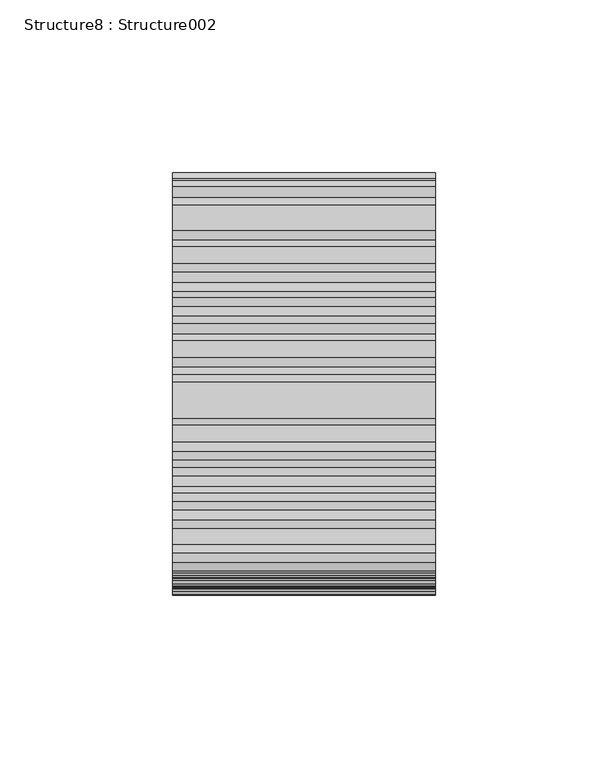
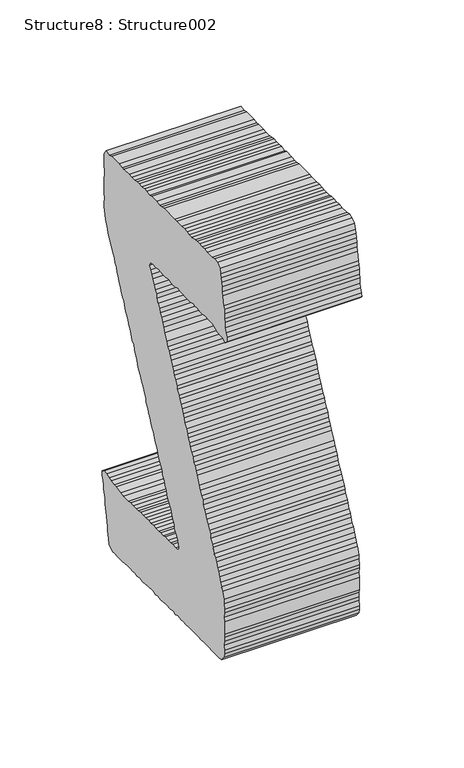
"""IFC4 building model written with IfcOpenShell, lengths in millimetres: proxy geometry, Structure8 : Structure002."""

from ifc_helpers import new_model, si_unit, frame, origin, place, context, project, spatial, polyline, outline, extrude, source, transform, mapped, element, save


def structure8_structure002_856189c6(model_context):
    return source(origin(), model_context, "Body", "SweptSolid", [
        extrude(outline(polyline([(2.492598, 0.0), (3.6086259, -2.5762556), (4.2959642, -5.0304922), (4.9764723, -7.4847267), (6.2027504, -9.6321841), (6.7842527, -12.5126982), (7.5898251, -14.5452844), (8.7003896, -17.1188063), (9.3874124, -19.5741986), (10.0456375, -21.3367914), (10.7326603, -23.7921837), (11.6960865, -26.0994951), (12.9542114, -28.9331331), (14.0275724, -30.8128021), (14.7236303, -33.2737663), (15.5292027, -35.3063524), (16.5191192, -38.292172), (14.6444913, -41.866959), (12.6028699, -42.6669596), (10.8807391, -44.0162015), (6.0473046, -46.7762723), (1.4407763, -48.6916737), (-0.4433067, -49.7675552), (-2.7074205, -51.4097046), (-5.0096886, -52.375129), (-6.3099559, -53.8327276), (-8.7690266, -54.5218508), (-11.1433905, -56.5927984), (-16.0213856, -58.6632174), (-20.0485121, -60.9628564), (-21.8924489, -62.7309104), (-24.0800527, -63.265016), (-26.1866282, -65.1830464), (-28.6055525, -66.5643422), (-30.9149624, -67.5172599), (-34.9457673, -69.8189993), (-37.510674, -70.9344002), (-39.0824083, -72.5470164), (-41.2744262, -73.0836426), (-43.6487901, -75.1545902), (-45.9574643, -76.1070878), (-48.219586, -77.7646846), (-50.5238461, -78.7146616), (-58.5869273, -83.3189807), (-61.110952, -85.1261339), (-62.8811066, -85.7711168), (-67.4519025, -88.3812112), (-69.4366719, -89.8804296), (-75.6193484, -93.4109677), (-78.4635995, -94.6692996), (-81.7199432, -93.3318287), (-83.4889419, -91.4845292), (-84.5581018, -89.6122169), (-85.4008779, -86.8857779), (-86.8984097, -84.8834606), (-88.1246878, -82.7360031), (-89.3170185, -81.2784046), (-93.0000537, -74.8286753), (-93.6857117, -72.3773815), (-95.753403, -70.0070116), (-96.6809884, -68.3826244), (-97.6720606, -65.3964894), (-98.9025397, -63.2416751), (-99.9709638, -58.8763448), (-100.0929769, -56.7919458), (-100.0855196, -54.3106986), (-100.5064322, -51.6926162), (-101.0804771, -48.823453), (-100.7731694, -46.8587615), (-101.3546716, -43.9782474), (-101.8848918, -41.7991562), (-101.3113735, -39.6873265), (-102.0372804, -36.5351385), (-102.2773205, -34.883003), (-101.8888818, -31.8183601), (-102.8432728, -29.5166206), (-102.8007104, -27.7187177), (-103.1167317, -24.670995), (-102.8433774, -22.0369352), (-103.1067517, -19.6947337), (-103.1096945, -17.2038161), (-103.1016019, -14.706597), (-104.2213082, -12.1324419), (-103.9075945, -10.1806771), (-104.0688112, -7.4142986), (-104.2129002, -4.648871), (-104.6411697, 0.4576085), (-104.9043371, 2.7891968), (-105.1715969, 5.1399108), (-104.8677605, 7.0918886), (-105.7105366, 9.8183277), (-105.2863656, 12.1882775), (-105.4431682, 14.9571766), (-105.9772738, 17.1447805), (-105.9730728, 19.6300217), (-106.087944, 21.701914), (-106.507914, 24.3098034), (-106.3936699, 27.2344558), (-106.8132196, 29.8416095), (-106.934497, 31.9264286), (-107.624569, 34.3752018), (-107.6189991, 36.8700049), (-107.7719163, 39.6303914), (-108.0012408, 41.2740122), (-107.6219398, 44.3529487), (-108.2634594, 46.1084961), (-108.3049706, 49.2973651), (-108.1557299, 51.5269043), (-108.6898354, 53.7145081), (-108.9617224, 56.0528242), (-108.9931492, 59.230867), (-109.2673436, 61.5834745), (-109.6852131, 64.1876855), (-109.1029752, 66.2927875), (-109.9522658, 69.0203844), (-109.9070742, 73.3182402), (-110.0641924, 76.0859834), (-110.9060258, 78.8022295), (-110.9060258, 81.2948275), (-110.4857403, 83.6732899), (-111.4405515, 85.975765), (-111.4469575, 88.4812897), (-111.168769, 91.1171345), (-112.1362938, 93.423081), (-111.8199509, 95.3822006), (-112.248536, 97.9949262), (-112.1278858, 100.9066519), (-112.3989325, 103.2434966), (-112.2482204, 105.473876), (-112.2375048, 107.9579594), (-114.8123895, 109.3509215), (-117.2703044, 108.6614827), (-119.381714, 106.7416673), (-121.8366863, 106.0539089), (-123.717091, 104.9801279), (-125.556298, 103.2157502), (-127.4403811, 102.1398688), (-130.1660845, 101.2975128), (-131.6278841, 100.1125389), (-133.6149652, 98.6139517), (-136.0331538, 97.2330761), (-138.2247516, 96.6957143), (-139.9543397, 95.3578231), (-142.6403168, 93.8240303), (-144.0925566, 92.6308574), (-148.6626168, 90.0211831), (-151.3846418, 89.1809277), (-152.4175408, 87.8769819), (-155.1476583, 87.0321053), (-156.9920151, 85.264787), (-158.8724198, 84.191006), (-161.8622333, 83.1978334), (-163.4373303, 81.5842724), (-167.197404, 79.4371305), (-169.2663536, 76.8313416), (-170.8404014, 75.2125263), (-172.8367266, 73.723294), (-174.5623268, 72.3681687), (-176.107991, 70.07778), (-178.9034826, 70.6082072), (-179.8629149, 72.9187748), (-180.1299677, 75.2588758), (-180.8181462, 77.7145837), (-182.0885647, 80.5509574), (-182.7393264, 82.3226899), (-184.2663976, 84.9968961), (-185.2279304, 87.3111421), (-185.6031329, 89.2187665), (-187.4147986, 94.2552506), (-187.9461746, 96.4346575), (-189.3341919, 98.8653527), (-190.2922614, 101.1649918), (-190.9779193, 103.6162856), (-191.3653068, 105.5384146), (-192.3538582, 108.5201355), (-191.1320927, 111.3777354), (-189.0208962, 113.2876734), (-186.570125, 113.9827886), (-182.534906, 116.2870487), (-180.6951764, 118.041969), (-178.1225991, 119.1558964), (-176.1251161, 120.6516434), (-173.9769229, 121.8783415), (-172.2077111, 122.5335173), (-169.3750159, 123.8018353), (-167.2246156, 125.0297938), (-165.4946074, 126.3669492), (-163.5000672, 127.8610157), (-160.9282256, 128.974523), (-156.6340464, 131.426659), (-155.1706689, 132.6174118), (-146.043055, 137.8296187), (-144.005319, 138.6381319), (-141.9752534, 139.4481184), (-139.8596428, 141.360577), (-135.5654635, 143.812713), (-133.6487978, 144.2028341), (-131.262456, 146.2698903), (-129.3827871, 147.3432512), (-126.8153596, 148.4542379), (-124.8164052, 149.950825), (-123.203789, 150.8716888), (-120.7486036, 151.5693247), (-118.0663049, 153.101017), (-116.0663013, 154.5923498), (-111.7713863, 157.044906), (-110.0091092, 157.7019753), (-107.8934986, 159.6144339), (-101.4474478, 163.2953686), (-99.2637293, 163.8379868), (-96.8766519, 165.905463), (-93.8797991, 164.4022527), (-92.5390698, 162.6762366), (-91.4234621, 160.1007166), (-90.3564027, 158.2320829), (-89.4027472, 155.9299233), (-88.0147299, 153.499228), (-86.405579, 151.9352707), (-85.1814014, 149.7914917), (-84.059072, 147.2042008), (-82.5721472, 145.2221671), (-81.8012598, 143.8721896), (-81.1179135, 141.421527), (-79.1945262, 139.3072791), (-78.0780782, 136.7302878), (-77.4365587, 134.9747404), (-75.9365062, 130.475411), (-75.6734474, 125.6394558), (-74.7127487, 123.3471717), (-74.6740758, 120.1547308), (-74.5645612, 118.0905108), (-74.8248924, 115.4336448), (-74.5574195, 113.0928082), (-74.5574195, 110.6002102), (-73.873233, 108.1480761), (-74.297404, 105.7781264), (-73.3383918, 103.4682944), (-73.2957248, 100.2791098), (-72.9115957, 98.3541447), (-72.7608835, 95.5993281), (-72.6442273, 93.5226015), (-72.3412291, 90.4976849), (-72.9197887, 88.3946833), (-72.1100172, 86.3479102), (-71.8115377, 83.3223644), (-72.2318232, 80.943902), (-71.9606719, 78.6051659), (-71.5380789, 75.9841408), (-71.3835838, 73.2295332), (-70.4331867, 68.4319394), (-71.2813216, 66.1740247), (-70.5812696, 63.7163169), (-70.3182109, 61.3729595), (-70.280165, 58.1918675), (-69.8978208, 56.2717365), (-69.4738569, 53.6671034), (-69.7421739, 51.010555), (-69.3637152, 49.0989367), (-69.368865, 46.603398), (-69.3684449, 44.1100642), (-68.9401754, 41.4961828), (-69.2116423, 38.8485672), (-68.4097483, 36.8138805), (-68.6387552, 33.4802914), (-68.1009712, 31.2947879), (-68.1000285, 28.791997), (-67.9471113, 26.0316105), (-67.6800586, 23.6915096), (-67.8379124, 21.4736367), (-67.2604042, 18.5898664), (-67.2648182, 16.0947478), (-67.0400124, 14.4504977), (-66.7614038, 12.1004108), (-66.3084292, 8.8128555), (-66.5727543, 6.1527332), (-66.3057015, 1.3200343), (-65.6572473, -0.4374066), (-66.0412719, -3.4995289), (-65.499709, -5.6984836), (-65.7722271, -8.3476751), (-64.8134219, -10.646894), (-64.5488918, -12.989411), (-64.9706487, -17.8613117), (-64.4002822, -20.7325754), (-64.2406434, -23.5047327), (-64.2443218, -25.9994313), (-63.4346508, -28.0306526), (-63.827188, -31.0966604), (-63.8586148, -32.9038136), (-63.2919267, -35.7771778), (-62.8999181, -37.7073993), (-61.4480986, -39.0060887), (-58.8729987, -37.8897452), (-56.6073071, -36.2418168), (-54.5788194, -35.4376092), (-52.4306263, -34.210911), (-50.1605206, -32.560462), (-47.9715519, -32.030455), (-45.9772186, -30.5257753), (-44.2114782, -29.8833131), (-41.9545062, -28.2286569), (-40.2229202, -26.8857226), (-37.230586, -25.8969641), (-35.9243268, -24.4310659), (-33.3573195, -23.3193436), (-31.2054479, -22.0905449), (-29.206809, -20.5951135), (-26.7537303, -19.9142899), (-25.2986523, -18.7175451), (-22.4507228, -17.4571126), (-20.8803535, -15.8403979), (-18.4199179, -15.1553732), (-14.1250029, -12.702817), (-12.2831667, -10.9310845), (-8.5683892, -8.0947109), (-7.1045916, -6.9046938), (-4.5757326, -5.0957556), (-3.2618089, -3.6518215), (-1.9989544, -1.4965871), (0.0, 0.0), (2.492598, 0.0)])), frame((-35624.0862846, 275201.6458391, 4026.4392678), z_axis=(1.0, 0.0, 1.354250045437766e-12), x_axis=(0.0, 0.8683895135052331, -0.4958827006804579)), (0.0, 0.0, 1.0), 76.2),
    ])


if __name__ == "__main__":
    model = new_model("IFC4")
    model_context = context("Model", 3, world=origin())
    ifc_project = project(units=[si_unit("LENGTHUNIT", "METRE", prefix="MILLI")], contexts=[model_context])
    site = spatial("IfcSite", under=ifc_project)
    building = spatial("IfcBuilding", under=site)
    placement = place(None, origin())
    structure8_structure002_shape = structure8_structure002_856189c6(model_context)
    element("IfcBuildingElementProxy", 1, Name="Structure8 : Structure002", ObjectType="Structure8 : Structure002", at=placement, inside=building, context=model_context, shape_type="MappedRepresentation", body=[
        mapped(structure8_structure002_shape, transform((0.0, 0.0, 0.0), x_axis=(1.0, 0.0, 0.0), y_axis=(0.0, 1.0, 0.0), z_axis=(0.0, 0.0, 1.0))),
    ])
    save(model, "model.ifc")

# Revit data of these elements
# Type "Structure8 : Structure002"
#   NameOverride = "Structure002"
# Element 1 (IfcBuildingElementProxy, "Structure8 : Structure002")
#   Materials on its faces: "BRUSHED ALUMINUM LETTERING"
# Materials
#   "BRUSHED ALUMINUM LETTERING": class "Unassigned", colour RGB 169 181 186, transparency 0, Cost = 0
